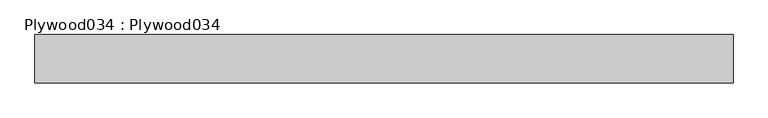
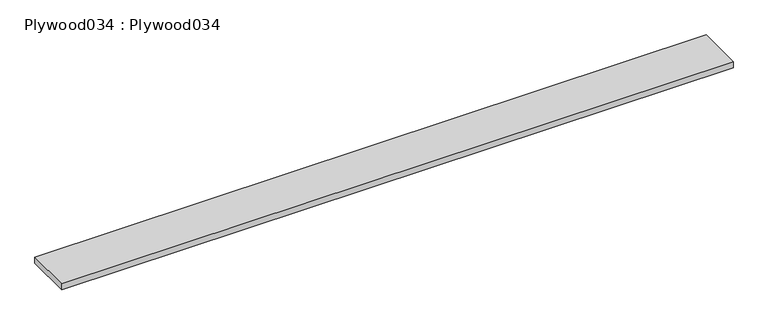
"""IFC4 building model written with IfcOpenShell, lengths in millimetres: proxy geometry, Plywood034 : Plywood034."""

from ifc_helpers import new_model, si_unit, frame, origin, place, context, project, spatial, polyline, outline, extrude, source, transform, mapped, element, save


def plywood034_plywood034_dee9376f(model_context):
    return source(origin(), model_context, "Body", "SweptSolid", [
        extrude(outline(polyline([(12382.7678845, -5363.3725586), (12382.7678845, -5224.4032789), (14383.0178845, -5224.4032789), (14383.0178845, -5363.3725586), (12382.7678845, -5363.3725586)])), frame((0.0, 0.0, 42642.0307603), z_axis=(0.0, 0.0, 1.0), x_axis=(1.0, 0.0, 0.0)), (0.0, 0.0, 1.0), 19.05),
    ])


if __name__ == "__main__":
    model = new_model("IFC4")
    model_context = context("Model", 3, world=origin())
    ifc_project = project(units=[si_unit("LENGTHUNIT", "METRE", prefix="MILLI")], contexts=[model_context])
    site = spatial("IfcSite", under=ifc_project)
    building = spatial("IfcBuilding", under=site)
    placement = place(None, origin())
    plywood034_plywood034_shape = plywood034_plywood034_dee9376f(model_context)
    element("IfcBuildingElementProxy", 1, Name="Plywood034 : Plywood034", ObjectType="Plywood034 : Plywood034", at=placement, inside=building, context=model_context, shape_type="MappedRepresentation", body=[
        mapped(plywood034_plywood034_shape, transform((0.0, 0.0, 0.0), x_axis=(1.0, 0.0, 0.0), y_axis=(0.0, 1.0, 0.0), z_axis=(0.0, 0.0, 1.0))),
    ])
    save(model, "model.ifc")

# Revit data of these elements
# Type "Plywood034 : Plywood034"
#   NameOverride = "Plywood034"
# Element 1 (IfcBuildingElementProxy, "Plywood034 : Plywood034")
#   Materials on its faces: "CDX PLYWOOD - SEE STRUCTURAL DWGS"
# Materials
#   "CDX PLYWOOD - SEE STRUCTURAL DWGS": class "Unassigned", colour RGB 177 130 114, transparency 0, Cost = 0
